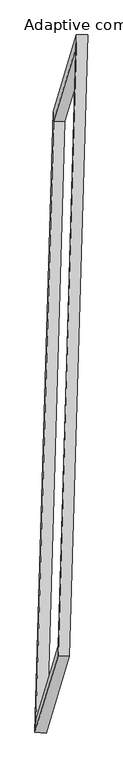
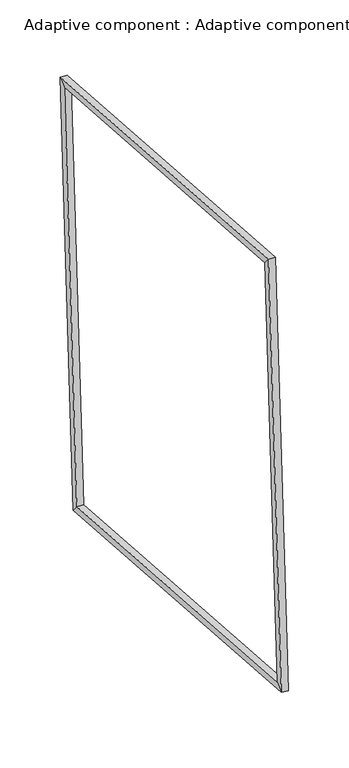
"""IFC4 building model written with IfcOpenShell, lengths in millimetres: proxy geometry, Adaptive component : Adaptive component."""

from ifc_helpers import new_model, si_unit, origin, place, context, project, spatial, faceted_brep, source, transform, mapped, element, save


def adaptive_component_adaptive_component_500e1eb8(model_context):
    return source(origin(), model_context, "Body", "Brep", [
        faceted_brep([(98.7026414, 1605.7520195, 3157.3619923), (163.7268091, 1605.6168574, 3157.0198145), (28.7354651, 1161.1032899, -870.272143), (-36.1681326, 1161.6354777, -866.3329134), (96.4423373, 1534.0204329, 3099.9495131), (-34.1013333, 1104.1526281, -794.6518656), (161.4665049, 1533.8852708, 3099.6073352), (30.8022643, 1103.6204404, -798.5910952), (-77.8133025, -2448.3285679, -468.3085878), (-142.6107151, -2444.1992704, -464.7699495), (-136.7330729, -2372.5865084, -407.4656051), (-71.9356603, -2376.7158058, -411.0042433), (57.1780415, -2003.8150004, 3558.9833697), (-7.7399411, -2000.0827286, 3558.9249562), (-6.1894023, -1942.7187036, 3487.1357737), (58.7285804, -1946.4509754, 3487.1941871)], [[[0, 1, 2, 3]], [[4, 0, 3, 5]], [[6, 4, 5, 7]], [[1, 6, 7, 2]], [[3, 2, 8, 9]], [[5, 3, 9, 10]], [[7, 5, 10, 11]], [[2, 7, 11, 8]], [[9, 8, 12, 13]], [[10, 9, 13, 14]], [[11, 10, 14, 15]], [[8, 11, 15, 12]], [[13, 12, 1, 0]], [[14, 13, 0, 4]], [[15, 14, 4, 6]], [[12, 15, 6, 1]]]),
    ])


if __name__ == "__main__":
    model = new_model("IFC4")
    model_context = context("Model", 3, world=origin())
    ifc_project = project(units=[si_unit("LENGTHUNIT", "METRE", prefix="MILLI")], contexts=[model_context])
    site = spatial("IfcSite", under=ifc_project)
    building = spatial("IfcBuilding", under=site)
    placement = place(None, origin())
    adaptive_component_adaptive_component_shape = adaptive_component_adaptive_component_500e1eb8(model_context)
    element("IfcBuildingElementProxy", 1, Name="Adaptive component : Adaptive component", ObjectType="Adaptive component : Adaptive component", at=placement, inside=building, context=model_context, shape_type="MappedRepresentation", body=[
        mapped(adaptive_component_adaptive_component_shape, transform((0.0, 0.0, 0.0), x_axis=(1.0, 0.0, 0.0), y_axis=(0.0, 1.0, 0.0), z_axis=(0.0, 0.0, 1.0))),
    ])
    save(model, "model.ifc")

# Revit data of these elements
# Type "Adaptive component : Adaptive component"
#   r [instance default] = 2063.125 mm
#   2r [instance default] = 4126.251 mm
#   Number [instance default] = 5
#   Default Elevation = 0
# Element 1 (IfcBuildingElementProxy, "Adaptive component : Adaptive component")
#   r = 2627.823 mm
#   2r = 5255.645 mm
#   Number = 25
